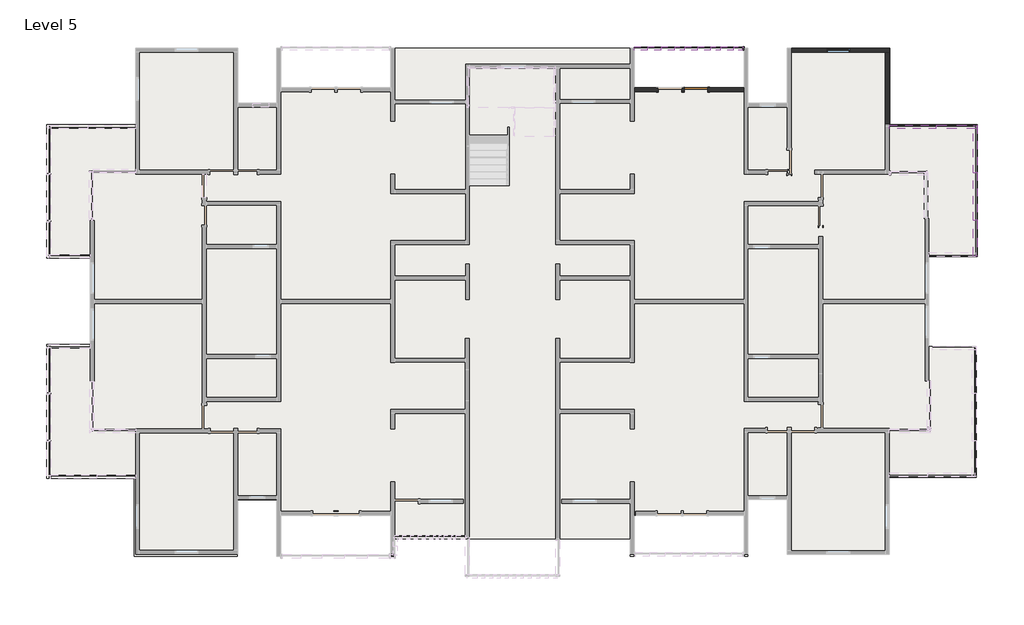
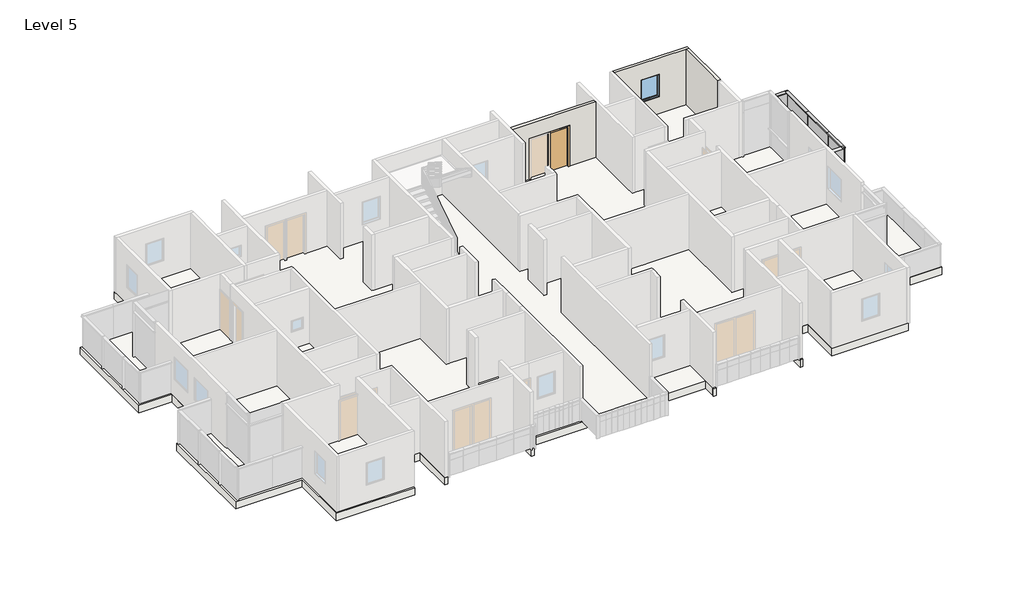
# One storey, part 5 of 7: 15 members, 14 plates, 3 walls, 1 door, 1 slab, 1 window.
"""IFC4 building model written with IfcOpenShell, lengths in millimetres."""

import ifcopenshell
import ifcopenshell.guid

model = None  # the IFC model being written
_history = None  # IfcOwnerHistory: only IFC2X3 demands one
_inside = {}  # id of a spatial element -> (the spatial element, [elements in it])
_under = {}  # id of a project, library or spatial element -> (it, [spatial elements below it])
_declared = {}  # id of a project -> (the project, [libraries it declares])
_typed = {}  # id of a type object -> (the type object, [elements of that type])
_made_of = {}  # id of a material, layer set ... -> (it, [elements and type objects made of it])


def new_model(schema):
    """Start an empty IFC model of exactly this schema.

    Asked for "IFC4X3", IfcOpenShell would pick the latest addendum, in which some entities
    have other attributes; the version numbers below select the first issue.
    IFC2X3 requires an IfcOwnerHistory on every rooted entity: one is made here for all.
    """
    global model, _history
    if schema == "IFC4X3":
        model = ifcopenshell.file(schema_version=(4, 3, 0, 0))
    else:
        model = ifcopenshell.file(schema=schema)
    _inside.clear()
    _under.clear()
    _declared.clear()
    _typed.clear()
    _made_of.clear()
    _history = None
    if model.schema == "IFC2X3":
        org = make("IfcOrganization", Name="unknown")
        user = make(
            "IfcPersonAndOrganization",
            ThePerson=make("IfcPerson", FamilyName="unknown"),
            TheOrganization=org,
        )
        app = make(
            "IfcApplication",
            ApplicationDeveloper=org,
            Version="unknown",
            ApplicationFullName="unknown",
            ApplicationIdentifier="unknown",
        )
        _history = make(
            "IfcOwnerHistory",
            OwningUser=user,
            OwningApplication=app,
            ChangeAction="ADDED",
            CreationDate=0,
        )
    return model


def make(cls, **values):
    """One entity of the class cls with the attributes given. An attribute that is None is left unset."""
    return model.create_entity(
        cls, **{name: value for name, value in values.items() if value is not None}
    )


def rooted(cls, **values):
    """An entity with a GlobalId (a new one), such as an element, a storey or a relation."""
    return make(cls, GlobalId=ifcopenshell.guid.new(), OwnerHistory=_history, **values)


def si_unit(unit_type, name, prefix=None):
    """IfcSIUnit, for example si_unit("LENGTHUNIT", "METRE", prefix="MILLI")."""
    return make("IfcSIUnit", UnitType=unit_type, Prefix=prefix, Name=name)


def assignment(units):
    """IfcUnitAssignment: the units of a project."""
    return None if units is None else make("IfcUnitAssignment", Units=units)


def point(xyz):
    """IfcCartesianPoint."""
    return None if xyz is None else make("IfcCartesianPoint", Coordinates=xyz)


def direction(xyz):
    """IfcDirection."""
    return None if xyz is None else make("IfcDirection", DirectionRatios=xyz)


def frame(location, z_axis=None, x_axis=None):
    """IfcAxis2Placement3D, a coordinate frame: its origin and axes. An axis left out is left unset."""
    return make(
        "IfcAxis2Placement3D",
        Location=point(location),
        Axis=direction(z_axis),
        RefDirection=direction(x_axis),
    )


def origin():
    """The frame at (0, 0, 0) with its axes left unset."""
    return frame((0.0, 0.0, 0.0))


def origin_with_axes():
    """The frame at (0, 0, 0) with the z axis (0, 0, 1) and the x axis (1, 0, 0) written out."""
    return frame((0.0, 0.0, 0.0), z_axis=(0.0, 0.0, 1.0), x_axis=(1.0, 0.0, 0.0))


def place(relative_to, where):
    """IfcLocalPlacement: puts the frame where relative to a parent placement (None: the world)."""
    return make(
        "IfcLocalPlacement", PlacementRelTo=relative_to, RelativePlacement=where
    )


def context(
    kind, dimensions, precision=None, world=None, true_north=None, identifier=None
):
    """IfcGeometricRepresentationContext, for example the 3D "Model" context."""
    return make(
        "IfcGeometricRepresentationContext",
        ContextIdentifier=identifier,
        ContextType=kind,
        CoordinateSpaceDimension=dimensions,
        Precision=precision,
        WorldCoordinateSystem=world,
        TrueNorth=true_north,
    )


def project(units=None, contexts=None):
    """IfcProject with its units and contexts."""
    return rooted(
        "IfcProject",
        Name="project",
        RepresentationContexts=contexts,
        UnitsInContext=assignment(units),
    )


def spatial(cls, under=None, at=None, **own):
    """A site, building, storey or space (cls), placed at a placement, below another one or the project."""
    s = rooted(cls, ObjectPlacement=at, **own)
    if under is not None:
        _under.setdefault(under.id(), (under, []))[1].append(s)
    return s


def polyline(points):
    """IfcPolyline through the points."""
    return make("IfcPolyline", Points=[point(p) for p in points])


def outline(outer, holes=None, kind="AREA"):
    """IfcArbitraryClosedProfileDef: a profile drawn as a closed curve; with holes, ...WithVoids."""
    if holes is None:
        return make("IfcArbitraryClosedProfileDef", ProfileType=kind, OuterCurve=outer)
    return make(
        "IfcArbitraryProfileDefWithVoids",
        ProfileType=kind,
        OuterCurve=outer,
        InnerCurves=holes,
    )


def extrude(swept, where, along, depth):
    """IfcExtrudedAreaSolid: the profile swept, set in the frame where, extruded along a direction by depth."""
    return make(
        "IfcExtrudedAreaSolid",
        SweptArea=swept,
        Position=where,
        ExtrudedDirection=direction(along),
        Depth=depth,
    )


def faces_of(points, faces, orient=None, outer=None):
    """IfcFace entities. A face is a list of loops; a loop is a list of indices into points, from 0.

    orient and outer hold one flag for each loop. By default every Orientation is true, the
    first loop of a face is its IfcFaceOuterBound and the others are IfcFaceBound.
    """
    made = []
    for i, loops in enumerate(faces):
        bounds = []
        for j, loop in enumerate(loops):
            is_outer = j == 0 if outer is None else outer[i][j]
            bounds.append(
                make(
                    "IfcFaceOuterBound" if is_outer else "IfcFaceBound",
                    Bound=make("IfcPolyLoop", Polygon=[points[k] for k in loop]),
                    Orientation=True if orient is None else orient[i][j],
                )
            )
        made.append(make("IfcFace", Bounds=bounds))
    return made


def faceted_brep(points, faces, orient=None, outer=None, voids=None):
    """IfcFacetedBrep: a solid bounded by flat faces; with voids (closed shells), ...WithVoids."""
    shared = [point(p) for p in points]
    hull = make("IfcClosedShell", CfsFaces=faces_of(shared, faces, orient, outer))
    if voids is None:
        return make("IfcFacetedBrep", Outer=hull)
    return make(
        "IfcFacetedBrepWithVoids",
        Outer=hull,
        Voids=[
            make(cls, CfsFaces=faces_of(shared, fs, o, b)) for cls, fs, o, b in voids
        ],
    )


def shape(context_of_items, identifier, shape_type, items):
    """IfcShapeRepresentation: the items that make up one representation, for example the "Body"."""
    return make(
        "IfcShapeRepresentation",
        ContextOfItems=context_of_items,
        RepresentationIdentifier=identifier,
        RepresentationType=shape_type,
        Items=items,
    )


def source(mapping_origin, context_of_items, identifier, shape_type, items):
    """IfcRepresentationMap: a shape defined once, which mapped items show again and again."""
    return make(
        "IfcRepresentationMap",
        MappingOrigin=mapping_origin,
        MappedRepresentation=shape(context_of_items, identifier, shape_type, items),
    )


def transform(
    local_origin,
    x_axis=None,
    y_axis=None,
    z_axis=None,
    scale=None,
    scale2=None,
    scale3=None,
    uniform=True,
):
    """IfcCartesianTransformationOperator3D, or its non-uniform kind. x_axis, y_axis, z_axis: its Axis1, 2, 3."""
    if uniform:
        return make(
            "IfcCartesianTransformationOperator3D",
            Axis1=direction(x_axis),
            Axis2=direction(y_axis),
            LocalOrigin=point(local_origin),
            Scale=scale,
            Axis3=direction(z_axis),
        )
    return make(
        "IfcCartesianTransformationOperator3DnonUniform",
        Axis1=direction(x_axis),
        Axis2=direction(y_axis),
        LocalOrigin=point(local_origin),
        Scale=scale,
        Axis3=direction(z_axis),
        Scale2=scale2,
        Scale3=scale3,
    )


def mapped(mapping_source, mapping_target):
    """IfcMappedItem: shows the shape of a source again, moved by a transform."""
    return make(
        "IfcMappedItem", MappingSource=mapping_source, MappingTarget=mapping_target
    )


def made_of(thing, what):
    """Note that an element or type object is made of a material, layer set ...; save() writes the relation."""
    if what is not None:
        _made_of.setdefault(what.id(), (what, []))[1].append(thing)
    return thing


def element(
    cls,
    number,
    at=None,
    inside=None,
    cuts=None,
    type_object=None,
    material=None,
    context=None,
    identifier="Body",
    shape_type=None,
    held_by="IfcProductDefinitionShape",
    body=None,
    shapes=None,
    **own,
):
    """One element of the class cls, such as IfcWall. Its Tag is "e" and its number.

    at: its placement. inside: the storey or other place that contains it. cuts: it is an
    opening in that element (IfcRelVoidsElement). A single representation is given by context,
    identifier, shape_type and body (its items); several are given by shapes. held_by: the class
    of the entity that holds the representations. save() writes the other relations.
    """
    e = rooted(cls, Tag="e%d" % number, ObjectPlacement=at, **own)
    if body is not None:
        shapes = [shape(context, identifier, shape_type, body)]
    if shapes is not None:
        e.Representation = make(held_by, Representations=shapes)
    if inside is not None:
        _inside.setdefault(inside.id(), (inside, []))[1].append(e)
    if cuts is not None:
        rooted(
            "IfcRelVoidsElement", RelatingBuildingElement=cuts, RelatedOpeningElement=e
        )
    if type_object is not None:
        _typed.setdefault(type_object.id(), (type_object, []))[1].append(e)
    return made_of(e, material)


def aggregate(whole, parts):
    """IfcRelAggregates: a whole, such as a stair, and the parts it consists of."""
    return rooted("IfcRelAggregates", RelatingObject=whole, RelatedObjects=parts)


def save(model, path):
    """Write the relations noted so far, then the file.

    IfcRelAggregates (storeys below a building ...), IfcRelContainedInSpatialStructure (elements
    in a storey), IfcRelDefinesByType, IfcRelAssociatesMaterial and IfcRelDeclares: one each for
    every whole, place, type object, material and project.
    """
    for whole, parts in _under.values():
        aggregate(whole, parts)
    for where, things in _inside.values():
        rooted(
            "IfcRelContainedInSpatialStructure",
            RelatedElements=things,
            RelatingStructure=where,
        )
    for kind, things in _typed.values():
        rooted("IfcRelDefinesByType", RelatedObjects=things, RelatingType=kind)
    for what, things in _made_of.values():
        rooted("IfcRelAssociatesMaterial", RelatedObjects=things, RelatingMaterial=what)
    for by, libraries in _declared.values():
        rooted("IfcRelDeclares", RelatingContext=by, RelatedDefinitions=libraries)
    model.write(path)


def m_single_flush_0915_x_2134mm_138fd904(model_context):
    return source(origin(), model_context, "Body", "SweptSolid", [
        extrude(outline(polyline([(2210.0, -533.5), (0.0, -533.5), (0.0, -457.5), (2134.0, -457.5), (2134.0, 457.5), (0.0, 457.5), (0.0, 533.5), (2210.0, 533.5), (2210.0, -533.5)])), frame((0.0, 75.0, 0.0), z_axis=(0.0, 1.0, 0.0), x_axis=(0.0, 0.0, 1.0)), (0.0, 0.0, 1.0), 25.0),
        extrude(outline(polyline([(2210.0, 533.5), (2210.0, -533.5), (0.0, -533.5), (0.0, -457.5), (2134.0, -457.5), (2134.0, 457.5), (0.0, 457.5), (0.0, 533.5), (2210.0, 533.5)])), frame((0.0, -100.0, 0.0), z_axis=(0.0, 1.0, 0.0), x_axis=(0.0, 0.0, 1.0)), (0.0, 0.0, 1.0), 25.0),
        extrude(outline(polyline([(457.5, 24.0), (-457.5, 24.0), (-457.5, 75.0), (457.5, 75.0), (457.5, 24.0)])), origin_with_axes(), (0.0, 0.0, 1.0), 2134.0),
    ])


def rectangular_mullion_50mm_x_150mm_42770ee2(model_context):
    return source(origin(), model_context, "Body", "SweptSolid", [
        extrude(outline(polyline([(0.0, 75.0), (0.0, -75.0), (-50.0, -75.0), (-50.0, 75.0), (0.0, 75.0)])), frame((0.0, 0.0, -1830.0000003), z_axis=(0.0, 0.0, 1.0), x_axis=(1.0, 0.0, 0.0)), (0.0, 0.0, 1.0), 1830.0000003),
    ])


def rectangular_mullion_50mm_x_150mm_aaee7d48(model_context):
    return source(origin(), model_context, "Body", "SweptSolid", [
        extrude(outline(polyline([(0.0, 75.0), (0.0, -75.0), (-50.0, -75.0), (-50.0, 75.0), (0.0, 75.0)])), frame((0.0, 0.0, -1830.0), z_axis=(0.0, 0.0, 1.0), x_axis=(1.0, 0.0, 0.0)), (0.0, 0.0, 1.0), 1830.0),
    ])


def rectangular_mullion_50mm_x_150mm_efa02866(model_context):
    return source(origin(), model_context, "Body", "SweptSolid", [
        extrude(outline(polyline([(0.0, 75.0), (0.0, -75.0), (-50.0, -75.0), (-50.0, 75.0), (0.0, 75.0)])), frame((0.0, 0.0, -1399.9999997), z_axis=(0.0, 0.0, 1.0), x_axis=(1.0, 0.0, 0.0)), (0.0, 0.0, 1.0), 1399.9999997),
    ])


def rectangular_mullion_50mm_x_150mm_d9f1e9e9(model_context):
    return source(origin(), model_context, "Body", "SweptSolid", [
        extrude(outline(polyline([(0.0, 75.0), (0.0, -75.0), (-50.0, -75.0), (-50.0, 75.0), (0.0, 75.0)])), frame((0.0, 0.0, -1565.8160321), z_axis=(0.0, 0.0, 1.0), x_axis=(1.0, 0.0, 0.0)), (0.0, 0.0, 1.0), 1565.8160321),
    ])


def rectangular_mullion_50mm_x_150mm_729c0cfc(model_context):
    return source(origin(), model_context, "Body", "SweptSolid", [
        extrude(outline(polyline([(0.0, 75.0), (0.0, -75.0), (-50.0, -75.0), (-50.0, 75.0), (0.0, 75.0)])), frame((0.0, 0.0, -1250.0), z_axis=(0.0, 0.0, 1.0), x_axis=(1.0, 0.0, 0.0)), (0.0, 0.0, 1.0), 1250.0),
    ])


def rectangular_mullion_50mm_x_150mm_b3666dbd(model_context):
    return source(origin(), model_context, "Body", "SweptSolid", [
        extrude(outline(polyline([(0.0, 75.0), (0.0, -75.0), (-50.0, -75.0), (-50.0, 75.0), (0.0, 75.0)])), frame((0.0, 0.0, -500.0), z_axis=(0.0, 0.0, 1.0), x_axis=(1.0, 0.0, 0.0)), (0.0, 0.0, 1.0), 500.0),
    ])


def rectangular_mullion_50mm_x_150mm_e851a0b8(model_context):
    return source(origin(), model_context, "Body", "SweptSolid", [
        extrude(outline(polyline([(0.0, 75.0), (0.0, -75.0), (-50.0, -75.0), (-50.0, 75.0), (0.0, 75.0)])), frame((0.0, 0.0, -522.7272727), z_axis=(0.0, 0.0, 1.0), x_axis=(1.0, 0.0, 0.0)), (0.0, 0.0, 1.0), 522.7272727),
    ])


def rectangular_mullion_50mm_x_150mm_e11a3e7b(model_context):
    return source(origin(), model_context, "Body", "SweptSolid", [
        extrude(outline(polyline([(0.0, 75.0), (0.0, -75.0), (-50.0, -75.0), (-50.0, 75.0), (0.0, 75.0)])), frame((0.0, 0.0, -400.0), z_axis=(0.0, 0.0, 1.0), x_axis=(1.0, 0.0, 0.0)), (0.0, 0.0, 1.0), 400.0),
    ])


def rectangular_mullion_50mm_x_150mm_23485ade(model_context):
    return source(origin(), model_context, "Body", "SweptSolid", [
        extrude(outline(polyline([(0.0, 75.0), (0.0, -75.0), (-50.0, -75.0), (-50.0, 75.0), (0.0, 75.0)])), frame((0.0, 0.0, -350.0), z_axis=(0.0, 0.0, 1.0), x_axis=(1.0, 0.0, 0.0)), (0.0, 0.0, 1.0), 350.0),
    ])


def system_panel_glazed_09fbcc53(model_context):
    return source(origin(), model_context, "Body", "SweptSolid", [
        extrude(outline(polyline([(915.0000002, 24.5), (-915.0000002, 24.5), (-915.0000002, 49.5), (915.0000002, 49.5), (915.0000002, 24.5)])), origin_with_axes(), (0.0, 0.0, 1.0), 1200.0),
    ])


def system_panel_glazed_f4bbd109(model_context):
    return source(origin(), model_context, "Body", "SweptSolid", [
        extrude(outline(polyline([(910.8343113, 24.5), (-910.8343113, 24.5), (-910.8343113, 49.5), (910.8343113, 49.5), (910.8343113, 24.5)])), origin_with_axes(), (0.0, 0.0, 1.0), 1200.0),
    ])


def system_panel_glazed_42eec186(model_context):
    return source(origin(), model_context, "Body", "SweptSolid", [
        extrude(outline(polyline([(699.9999998, 24.5), (-699.9999998, 24.5), (-699.9999998, 49.5), (699.9999998, 49.5), (699.9999998, 24.5)])), origin_with_axes(), (0.0, 0.0, 1.0), 1200.0),
    ])


def system_panel_glazed_f2fc581d(model_context):
    return source(origin(), model_context, "Body", "SweptSolid", [
        extrude(outline(polyline([(782.9080161, 24.5), (-782.9080161, 24.5), (-782.9080161, 49.5), (782.9080161, 49.5), (782.9080161, 24.5)])), origin_with_axes(), (0.0, 0.0, 1.0), 1200.0),
    ])


def system_panel_glazed_346501af(model_context):
    return source(origin(), model_context, "Body", "SweptSolid", [
        extrude(outline(polyline([(250.0, 24.5), (-250.0, 24.5), (-250.0, 49.5), (250.0, 49.5), (250.0, 24.5)])), origin_with_axes(), (0.0, 0.0, 1.0), 1200.0),
    ])


def system_panel_glazed_5241e6d5(model_context):
    return source(origin(), model_context, "Body", "SweptSolid", [
        extrude(outline(polyline([(261.3636364, 24.5), (-261.3636364, 24.5), (-261.3636364, 49.5), (261.3636364, 49.5), (261.3636364, 24.5)])), origin_with_axes(), (0.0, 0.0, 1.0), 1200.0),
    ])


def system_panel_glazed_3e660766(model_context):
    return source(origin(), model_context, "Body", "SweptSolid", [
        extrude(outline(polyline([(200.0, 24.5), (-200.0, 24.5), (-200.0, 49.5), (200.0, 49.5), (200.0, 24.5)])), origin_with_axes(), (0.0, 0.0, 1.0), 1200.0),
    ])


def system_panel_glazed_b0a6d7cd(model_context):
    return source(origin(), model_context, "Body", "SweptSolid", [
        extrude(outline(polyline([(175.0, 24.5), (-175.0, 24.5), (-175.0, 49.5), (175.0, 49.5), (175.0, 24.5)])), origin_with_axes(), (0.0, 0.0, 1.0), 1200.0),
    ])


def m_fixed_0915_x_1220mm_873aa0e2(model_context):
    return source(origin(), model_context, "Body", "SweptSolid", [
        extrude(outline(polyline([(-394.5, 53.0), (394.5, 53.0), (394.5, 41.0), (-394.5, 41.0), (-394.5, 53.0)])), frame((0.0, 0.0, 978.0), z_axis=(0.0, 0.0, 1.0), x_axis=(1.0, 0.0, 0.0)), (0.0, 0.0, 1.0), 1094.0),
        extrude(outline(polyline([(2116.0, -438.5), (934.0, -438.5), (934.0, 438.5), (2116.0, 438.5), (2116.0, -438.5)]), holes=[polyline([(2072.0, -394.5), (2072.0, 394.5), (978.0, 394.5), (978.0, -394.5), (2072.0, -394.5)])]), frame((0.0, 25.0, 0.0), z_axis=(0.0, 1.0, 0.0), x_axis=(0.0, 0.0, 1.0)), (0.0, 0.0, 1.0), 44.0),
        extrude(outline(polyline([(2135.0, -457.5), (915.0, -457.5), (915.0, 457.5), (2135.0, 457.5), (2135.0, -457.5)]), holes=[polyline([(2116.0, -438.5), (2116.0, 438.5), (934.0, 438.5), (934.0, -438.5), (2116.0, -438.5)])]), frame((0.0, 25.0, 0.0), z_axis=(0.0, 1.0, 0.0), x_axis=(0.0, 0.0, 1.0)), (0.0, 0.0, 1.0), 63.0),
        extrude(outline(polyline([(2135.0, -457.5), (915.0, -457.5), (915.0, 457.5), (2135.0, 457.5), (2135.0, -457.5)]), holes=[polyline([(2103.0, -425.5), (2103.0, 425.5), (947.0, 425.5), (947.0, -425.5), (2103.0, -425.5)])]), frame((0.0, -62.0, 0.0), z_axis=(0.0, 1.0, 0.0), x_axis=(0.0, 0.0, 1.0)), (0.0, 0.0, 1.0), 87.0),
    ])


model = new_model("IFC4")

# Units and contexts
model_context = context("Model", 3, world=origin())
ifc_project = project(units=[si_unit("LENGTHUNIT", "METRE", prefix="MILLI")], contexts=[model_context])

# Site, building, storey
site = spatial("IfcSite", under=ifc_project)
building = spatial("IfcBuilding", under=site)
storey = spatial("IfcBuildingStorey", under=building, Name="Level 5", Elevation=12500.0)

# Door
placement = place(None, origin())
m_single_flush_0915_x_2134mm_shape = m_single_flush_0915_x_2134mm_138fd904(model_context)
element("IfcDoor", 1, ObjectType="M_Single-Flush : 0915 x 2134mm", at=placement, inside=storey, context=model_context, shape_type="MappedRepresentation", body=[
    mapped(m_single_flush_0915_x_2134mm_shape, transform((6794.6515415, 8016.5690894, 12500.0), x_axis=(1.0, 0.0, 0.0), y_axis=(0.0, 1.0, 0.0), z_axis=(0.0, 0.0, 1.0))),
])

# Members
rectangular_mullion_50mm_x_150mm_shape = rectangular_mullion_50mm_x_150mm_42770ee2(model_context)
element("IfcMember", 2, ObjectType="Rectangular Mullion : 50mm x 150mm", at=placement, inside=storey, context=model_context, shape_type="MappedRepresentation", body=[
    mapped(rectangular_mullion_50mm_x_150mm_shape, transform((17635.0130284, 4788.3418163, 13750.0), x_axis=(0.0, 0.0, 1.0), y_axis=(-1.0, 0.0, 0.0), z_axis=(0.0, -1.0, 0.0))),
])
element("IfcMember", 3, ObjectType="Rectangular Mullion : 50mm x 150mm", at=placement, inside=storey, context=model_context, shape_type="MappedRepresentation", body=[
    mapped(rectangular_mullion_50mm_x_150mm_shape, transform((16129.1969963, 6568.8418166, 13750.0), x_axis=(0.0, 0.0, 1.0), y_axis=(0.0, -1.0, 0.0), z_axis=(1.0, 0.0, 0.0))),
])
rectangular_mullion_50mm_x_150mm_2_shape = rectangular_mullion_50mm_x_150mm_aaee7d48(model_context)
element("IfcMember", 4, ObjectType="Rectangular Mullion : 50mm x 150mm", at=placement, inside=storey, context=model_context, shape_type="MappedRepresentation", body=[
    mapped(rectangular_mullion_50mm_x_150mm_2_shape, transform((17635.0130284, 2958.3418163, 13750.0), x_axis=(0.0, 0.0, 1.0), y_axis=(-1.0, 0.0, 0.0), z_axis=(0.0, -1.0, 0.0))),
])
rectangular_mullion_50mm_x_150mm_3_shape = rectangular_mullion_50mm_x_150mm_efa02866(model_context)
element("IfcMember", 5, ObjectType="Rectangular Mullion : 50mm x 150mm", at=placement, inside=storey, context=model_context, shape_type="MappedRepresentation", body=[
    mapped(rectangular_mullion_50mm_x_150mm_3_shape, transform((17635.0130284, 1558.3418166, 13750.0), x_axis=(0.0, 0.0, 1.0), y_axis=(-1.0, 0.0, 0.0), z_axis=(0.0, -1.0, 0.0))),
])
rectangular_mullion_50mm_x_150mm_4_shape = rectangular_mullion_50mm_x_150mm_d9f1e9e9(model_context)
element("IfcMember", 6, ObjectType="Rectangular Mullion : 50mm x 150mm", at=placement, inside=storey, context=model_context, shape_type="MappedRepresentation", body=[
    mapped(rectangular_mullion_50mm_x_150mm_4_shape, transform((17695.0130284, 6568.8418166, 13750.0), x_axis=(0.0, 0.0, 1.0), y_axis=(0.0, -1.0, 0.0), z_axis=(1.0, 0.0, 0.0))),
])
rectangular_mullion_50mm_x_150mm_5_shape = rectangular_mullion_50mm_x_150mm_729c0cfc(model_context)
element("IfcMember", 7, ObjectType="Rectangular Mullion : 50mm x 150mm", at=placement, inside=storey, context=model_context, shape_type="MappedRepresentation", body=[
    mapped(rectangular_mullion_50mm_x_150mm_5_shape, transform((8667.3788142, 9614.2963621, 12500.0), x_axis=(1.0, 0.0, 0.0), y_axis=(0.0, -1.0, 0.0), z_axis=(0.0, 0.0, -1.0))),
])
rectangular_mullion_50mm_x_150mm_6_shape = rectangular_mullion_50mm_x_150mm_b3666dbd(model_context)
element("IfcMember", 8, ObjectType="Rectangular Mullion : 50mm x 150mm", at=placement, inside=storey, context=model_context, shape_type="MappedRepresentation", body=[
    mapped(rectangular_mullion_50mm_x_150mm_6_shape, transform((6867.3788142, 9614.2963621, 13750.0), x_axis=(0.0, 0.0, 1.0), y_axis=(0.0, -1.0, 0.0), z_axis=(1.0, 0.0, 0.0))),
])
element("IfcMember", 9, ObjectType="Rectangular Mullion : 50mm x 150mm", at=placement, inside=storey, context=model_context, shape_type="MappedRepresentation", body=[
    mapped(rectangular_mullion_50mm_x_150mm_6_shape, transform((7367.3788142, 9614.2963621, 13750.0), x_axis=(0.0, 0.0, 1.0), y_axis=(0.0, -1.0, 0.0), z_axis=(1.0, 0.0, 0.0))),
])
element("IfcMember", 10, ObjectType="Rectangular Mullion : 50mm x 150mm", at=placement, inside=storey, context=model_context, shape_type="MappedRepresentation", body=[
    mapped(rectangular_mullion_50mm_x_150mm_6_shape, transform((8267.3788142, 9614.2963621, 13750.0), x_axis=(0.0, 0.0, 1.0), y_axis=(0.0, -1.0, 0.0), z_axis=(1.0, 0.0, 0.0))),
])
rectangular_mullion_50mm_x_150mm_7_shape = rectangular_mullion_50mm_x_150mm_e851a0b8(model_context)
element("IfcMember", 11, ObjectType="Rectangular Mullion : 50mm x 150mm", at=placement, inside=storey, context=model_context, shape_type="MappedRepresentation", body=[
    mapped(rectangular_mullion_50mm_x_150mm_7_shape, transform((4921.9242687, 9614.2963621, 13750.0), x_axis=(0.0, 0.0, 1.0), y_axis=(0.0, -1.0, 0.0), z_axis=(1.0, 0.0, 0.0))),
])
element("IfcMember", 12, ObjectType="Rectangular Mullion : 50mm x 150mm", at=placement, inside=storey, context=model_context, shape_type="MappedRepresentation", body=[
    mapped(rectangular_mullion_50mm_x_150mm_7_shape, transform((5444.6515415, 9614.2963621, 13750.0), x_axis=(0.0, 0.0, 1.0), y_axis=(0.0, -1.0, 0.0), z_axis=(1.0, 0.0, 0.0))),
])
element("IfcMember", 13, ObjectType="Rectangular Mullion : 50mm x 150mm", at=placement, inside=storey, context=model_context, shape_type="MappedRepresentation", body=[
    mapped(rectangular_mullion_50mm_x_150mm_7_shape, transform((5967.3788142, 9614.2963621, 13750.0), x_axis=(0.0, 0.0, 1.0), y_axis=(0.0, -1.0, 0.0), z_axis=(1.0, 0.0, 0.0))),
])
rectangular_mullion_50mm_x_150mm_8_shape = rectangular_mullion_50mm_x_150mm_e11a3e7b(model_context)
element("IfcMember", 14, ObjectType="Rectangular Mullion : 50mm x 150mm", at=placement, inside=storey, context=model_context, shape_type="MappedRepresentation", body=[
    mapped(rectangular_mullion_50mm_x_150mm_8_shape, transform((6367.3788142, 9614.2963621, 13750.0), x_axis=(0.0, 0.0, 1.0), y_axis=(0.0, -1.0, 0.0), z_axis=(1.0, 0.0, 0.0))),
])
element("IfcMember", 15, ObjectType="Rectangular Mullion : 50mm x 150mm", at=placement, inside=storey, context=model_context, shape_type="MappedRepresentation", body=[
    mapped(rectangular_mullion_50mm_x_150mm_8_shape, transform((7767.3788142, 9614.2963621, 13750.0), x_axis=(0.0, 0.0, 1.0), y_axis=(0.0, -1.0, 0.0), z_axis=(1.0, 0.0, 0.0))),
])
rectangular_mullion_50mm_x_150mm_9_shape = rectangular_mullion_50mm_x_150mm_23485ade(model_context)
element("IfcMember", 16, ObjectType="Rectangular Mullion : 50mm x 150mm", at=placement, inside=storey, context=model_context, shape_type="MappedRepresentation", body=[
    mapped(rectangular_mullion_50mm_x_150mm_9_shape, transform((8617.3788142, 9614.2963621, 13750.0), x_axis=(0.0, 0.0, 1.0), y_axis=(0.0, -1.0, 0.0), z_axis=(1.0, 0.0, 0.0))),
])

# Plates
system_panel_glazed_shape = system_panel_glazed_09fbcc53(model_context)
element("IfcPlate", 17, ObjectType="System Panel : Glazed", at=placement, inside=storey, context=model_context, shape_type="MappedRepresentation", body=[
    mapped(system_panel_glazed_shape, transform((17635.0130284, 5703.3418165, 12500.0), x_axis=(0.0, -1.0, 0.0), y_axis=(1.0, 0.0, 0.0), z_axis=(0.0, 0.0, 1.0))),
])
element("IfcPlate", 18, ObjectType="System Panel : Glazed", at=placement, inside=storey, context=model_context, shape_type="MappedRepresentation", body=[
    mapped(system_panel_glazed_shape, transform((17635.0130284, 3873.3418163, 12500.0), x_axis=(0.0, -1.0, 0.0), y_axis=(1.0, 0.0, 0.0), z_axis=(0.0, 0.0, 1.0))),
])
system_panel_glazed_2_shape = system_panel_glazed_f4bbd109(model_context)
element("IfcPlate", 19, ObjectType="System Panel : Glazed", at=placement, inside=storey, context=model_context, shape_type="MappedRepresentation", body=[
    mapped(system_panel_glazed_2_shape, transform((16748.6787171, 1608.3418166, 12500.0), x_axis=(-1.0, 0.0, 0.0), y_axis=(0.0, -1.0, 0.0), z_axis=(0.0, 0.0, 1.0))),
])
system_panel_glazed_3_shape = system_panel_glazed_42eec186(model_context)
element("IfcPlate", 20, ObjectType="System Panel : Glazed", at=placement, inside=storey, context=model_context, shape_type="MappedRepresentation", body=[
    mapped(system_panel_glazed_3_shape, transform((17635.0130284, 2258.3418165, 12500.0), x_axis=(0.0, -1.0, 0.0), y_axis=(1.0, 0.0, 0.0), z_axis=(0.0, 0.0, 1.0))),
])
system_panel_glazed_4_shape = system_panel_glazed_f2fc581d(model_context)
element("IfcPlate", 21, ObjectType="System Panel : Glazed", at=placement, inside=storey, context=model_context, shape_type="MappedRepresentation", body=[
    mapped(system_panel_glazed_4_shape, transform((16912.1050124, 6568.8418166, 12500.0), x_axis=(1.0, 0.0, 0.0), y_axis=(0.0, 1.0, 0.0), z_axis=(0.0, 0.0, 1.0))),
])
system_panel_glazed_5_shape = system_panel_glazed_346501af(model_context)
element("IfcPlate", 22, ObjectType="System Panel : Glazed", at=placement, inside=storey, context=model_context, shape_type="MappedRepresentation", body=[
    mapped(system_panel_glazed_5_shape, transform((8017.3788142, 9614.2963621, 12500.0), x_axis=(1.0, 0.0, 0.0), y_axis=(0.0, 1.0, 0.0), z_axis=(0.0, 0.0, 1.0))),
])
element("IfcPlate", 23, ObjectType="System Panel : Glazed", at=placement, inside=storey, context=model_context, shape_type="MappedRepresentation", body=[
    mapped(system_panel_glazed_5_shape, transform((7117.3788142, 9614.2963621, 12500.0), x_axis=(1.0, 0.0, 0.0), y_axis=(0.0, 1.0, 0.0), z_axis=(0.0, 0.0, 1.0))),
])
element("IfcPlate", 24, ObjectType="System Panel : Glazed", at=placement, inside=storey, context=model_context, shape_type="MappedRepresentation", body=[
    mapped(system_panel_glazed_5_shape, transform((6617.3788142, 9614.2963621, 12500.0), x_axis=(1.0, 0.0, 0.0), y_axis=(0.0, 1.0, 0.0), z_axis=(0.0, 0.0, 1.0))),
])
system_panel_glazed_6_shape = system_panel_glazed_5241e6d5(model_context)
element("IfcPlate", 25, ObjectType="System Panel : Glazed", at=placement, inside=storey, context=model_context, shape_type="MappedRepresentation", body=[
    mapped(system_panel_glazed_6_shape, transform((4660.5606324, 9614.2963621, 12500.0), x_axis=(1.0, 0.0, 0.0), y_axis=(0.0, 1.0, 0.0), z_axis=(0.0, 0.0, 1.0))),
])
element("IfcPlate", 26, ObjectType="System Panel : Glazed", at=placement, inside=storey, context=model_context, shape_type="MappedRepresentation", body=[
    mapped(system_panel_glazed_6_shape, transform((5706.0151778, 9614.2963621, 12500.0), x_axis=(1.0, 0.0, 0.0), y_axis=(0.0, 1.0, 0.0), z_axis=(0.0, 0.0, 1.0))),
])
element("IfcPlate", 27, ObjectType="System Panel : Glazed", at=placement, inside=storey, context=model_context, shape_type="MappedRepresentation", body=[
    mapped(system_panel_glazed_6_shape, transform((5183.2879051, 9614.2963621, 12500.0), x_axis=(1.0, 0.0, 0.0), y_axis=(0.0, 1.0, 0.0), z_axis=(0.0, 0.0, 1.0))),
])
system_panel_glazed_7_shape = system_panel_glazed_3e660766(model_context)
element("IfcPlate", 28, ObjectType="System Panel : Glazed", at=placement, inside=storey, context=model_context, shape_type="MappedRepresentation", body=[
    mapped(system_panel_glazed_7_shape, transform((7567.3788142, 9614.2963621, 12500.0), x_axis=(1.0, 0.0, 0.0), y_axis=(0.0, 1.0, 0.0), z_axis=(0.0, 0.0, 1.0))),
])
element("IfcPlate", 29, ObjectType="System Panel : Glazed", at=placement, inside=storey, context=model_context, shape_type="MappedRepresentation", body=[
    mapped(system_panel_glazed_7_shape, transform((6167.3788142, 9614.2963621, 12500.0), x_axis=(1.0, 0.0, 0.0), y_axis=(0.0, 1.0, 0.0), z_axis=(0.0, 0.0, 1.0))),
])
system_panel_glazed_8_shape = system_panel_glazed_b0a6d7cd(model_context)
element("IfcPlate", 30, ObjectType="System Panel : Glazed", at=placement, inside=storey, context=model_context, shape_type="MappedRepresentation", body=[
    mapped(system_panel_glazed_8_shape, transform((8442.3788142, 9614.2963621, 12500.0), x_axis=(1.0, 0.0, 0.0), y_axis=(0.0, 1.0, 0.0), z_axis=(0.0, 0.0, 1.0))),
])

# Slab
element("IfcSlab", 31, ObjectType="Generic Floor - 400mm", at=placement, inside=storey, context=model_context, shape_type="SweptSolid", body=[
    extrude(outline(polyline([(-10978.0757313, 7482.4781803), (-9455.3484585, 7482.4781803), (-9455.3484585, 9614.2963621), (-9305.3484585, 9614.2963621), (-9305.3484585, 8091.5690894), (-5039.4393676, 8091.5690894), (-5039.4393676, 9614.2963621), (4399.196996, 9614.2963621), (4399.196996, 8091.5690894), (8665.1060869, 8091.5690894), (8665.1060869, 9614.2963621), (8817.3788142, 9614.2963621), (8817.3788142, 7482.4781803), (10342.3783683, 7482.4781803), (10342.3783683, 9614.2963621), (14312.8444058, 9614.2963621), (14312.8444058, 6653.3418166), (17717.8444058, 6653.3418166), (17717.8444058, 1533.3418166), (15837.8444058, 1533.3418166), (15837.8444058, -1946.1581834), (17677.8444058, -1946.1581834), (17677.8444058, -7028.8854561), (14240.1060869, -7028.8854561), (14240.1060869, -10028.8854561), (10340.1060869, -10028.8854561), (10340.1060869, -7894.794547), (8815.1060869, -7894.794547), (8815.1060869, -10106.1581834), (8665.1060869, -10106.1581834), (8665.1060869, -8506.1581834), (4401.4697233, -8506.1581834), (4401.4697233, -10106.1581834), (4251.4697233, -10106.1581834), (4251.4697233, -10028.8854561), (4251.4697233, -9417.5218198), (-4887.1666404, -9417.5218198), (-4887.1666404, -10006.7413208), (-4887.1666404, -10106.1581834), (-5039.4393676, -10106.1581834), (-5039.4393676, -8503.8854561), (-9303.0757313, -8503.8854561), (-9303.0757313, -10106.1581834), (-9453.0757313, -10106.1581834), (-9453.0757313, -7906.1581834), (-10989.3512663, -7906.1581834), (-10989.3512663, -10106.1581834), (-14989.3512663, -10106.1581834), (-14989.3512663, -7083.4309107), (-18389.3512663, -7083.4309107), (-18389.3512663, -1883.4309107), (-16697.1666404, -1883.4309107), (-16697.1666404, 1474.2963621), (-18377.1666404, 1474.2963621), (-18377.1666404, 6654.2963621), (-14937.1666404, 6654.2963621), (-14937.1666404, 9614.2963621), (-10978.0757313, 9614.2963621), (-10978.0757313, 7482.4781803)])), frame((0.0, 0.0, 12100.0), z_axis=(0.0, 0.0, 1.0), x_axis=(1.0, 0.0, 0.0)), (0.0, 0.0, 1.0), 400.0),
])

# Walls
element("IfcWall", 32, ObjectType="wal 150", at=placement, inside=storey, context=model_context, shape_type="SweptSolid", body=[
    extrude(outline(polyline([(12500.0, 8665.1060869), (15500.0, 8665.1060869), (15500.0, 4399.196996), (12500.0, 4399.196996), (12500.0, 5337.1515415), (14634.0, 5337.1515415), (14634.0, 6252.1515415), (12500.0, 6252.1515415), (12500.0, 6337.1515415), (14634.0, 6337.1515415), (14634.0, 7252.1515415), (12500.0, 7252.1515415), (12500.0, 8665.1060869)])), frame((0.0, 7941.5690894, 0.0), z_axis=(0.0, 1.0, 0.0), x_axis=(0.0, 0.0, 1.0)), (0.0, 0.0, 1.0), 150.0),
])
element("IfcWall", 33, ObjectType="wal 150", at=placement, inside=storey, context=model_context, shape_type="Brep", body=[
    faceted_brep([(10492.3783683, 9464.2963621, 12500.0), (14149.196996, 9464.2963621, 12500.0), (14299.196996, 9464.2963621, 12500.0), (14299.196996, 9464.2963621, 15500.0), (14149.196996, 9464.2963621, 15500.0), (10492.3783683, 9464.2963621, 15500.0), (11863.2876822, 9464.2963621, 13415.0), (11863.2876822, 9464.2963621, 14635.0), (12778.2876822, 9464.2963621, 14635.0), (12778.2876822, 9464.2963621, 13415.0), (10492.3783683, 9614.2963621, 12500.0), (10492.3783683, 9614.2963621, 15500.0), (14299.196996, 9614.2963621, 15500.0), (14299.196996, 9614.2963621, 12500.0), (11863.2876822, 9614.2963621, 13415.0), (12778.2876822, 9614.2963621, 13415.0), (12778.2876822, 9614.2963621, 14635.0), (11863.2876822, 9614.2963621, 14635.0)], [[[0, 1, 2, 3, 4, 5], [6, 7, 8, 9]], [[10, 11, 12, 13], [14, 15, 16, 17]], [[2, 1, 0, 10, 13]], [[5, 4, 3, 12, 11]], [[7, 6, 14, 17]], [[8, 7, 17, 16]], [[9, 8, 16, 15]], [[6, 9, 15, 14]], [[0, 5, 11, 10]], [[3, 2, 13, 12]]]),
])
element("IfcWall", 34, ObjectType="wal 150", at=placement, inside=storey, context=model_context, shape_type="SweptSolid", body=[
    extrude(outline(polyline([(14149.196996, 6668.8418166), (14149.196996, 9464.2963621), (14299.196996, 9464.2963621), (14299.196996, 6668.8418166), (14149.196996, 6668.8418166)])), frame((0.0, 0.0, 12500.0), z_axis=(0.0, 0.0, 1.0), x_axis=(1.0, 0.0, 0.0)), (0.0, 0.0, 1.0), 3000.0),
])

# Window
m_fixed_0915_x_1220mm_shape = m_fixed_0915_x_1220mm_873aa0e2(model_context)
element("IfcWindow", 35, ObjectType="M_Fixed : 1.80 to 1.20 w2", at=placement, inside=storey, context=model_context, shape_type="MappedRepresentation", body=[
    mapped(m_fixed_0915_x_1220mm_shape, transform((12320.7876822, 9526.2963621, 12500.0), x_axis=(1.0, 0.0, 0.0), y_axis=(0.0, 1.0, 0.0), z_axis=(0.0, 0.0, 1.0))),
])

save(model, "model.ifc")

# Revit data of these elements
# Type "M_Single-Flush : 0915 x 2134mm"
#   Type Mark = "15"
#   Thickness = 0.051 m
#   Height = 2.134 m
#   Trim Projection Ext = 0.025 m
#   Trim Projection Int = 0.025 m
#   Trim Width = 0.076 m
#   Width = 0.915 m
#   Door Material = Door - Panel
#   Frame Material = Door - Frame
#   Function = (empty or 0)
#   Wall Closure = (empty or 0)
# Type "Rectangular Mullion : 50mm x 150mm"
#   built-in parameter 1007304 = 0.492126 (stored number, unit not read)
#   built-in parameter 1007301 = 0.082021 (stored number, unit not read)
#   built-in parameter 1007300 = 0.082021 (stored number, unit not read)
# Type "Generic Floor - 400mm"
#   Function = 0
#   Layers, outside or top first: 0.4 m no material (function 1)
# Type "wal 150"
#   Layers, outside or top first: 0.15 m no material (function 1)
# Type "M_Fixed : 1.80 to 1.20 w2"
#   Type Mark = "19"
#   Height = 1.22 m
#   Default Sill Height = 0.915 m
#   Width = 0.915 m
#   Window Inset = 0.019 m
#   Frame Exterior Material = Sash
#   Frame Interior Material = Sash
#   Glass Pane Material = Glass
#   Sash = Sash
#   Wall Closure = (empty or 0)
# Element 1 (IfcDoor, "M_Single-Flush : 0915 x 2134mm")
#   Phase Created = New Construction
#   Materials on its faces: "Door - Frame", "Door - Panel"
# Elements 2, 3, 4, 5, 6, 7, 8, 9, 10, 11, 12, 13, 14, 15, 16 (IfcMember, "Rectangular Mullion : 50mm x 150mm")
#   Phase Created = New Construction
#   Materials on its faces: "Aluminum"
# Elements 17, 18, 19, 20, 21, 22, 23, 24, 25, 26, 27, 28, 29, 30 (IfcPlate, "System Panel : Glazed")
#   Phase Created = New Construction
#   Materials on its faces: "Glass"
# Element 31 (IfcSlab, "Generic Floor - 400mm")
#   built-in parameter 1001955 = 3.14159 (stored number, unit not read)
#   Height Offset From Level = 0 m
#   Phase Created = New Construction
#   Materials on its faces: "Default Roof", "Door - Frame", "Ceiling Tile 600 x 1200", "Oak Flooring"
# Element 32 (IfcWall, "wal 150")
#   Top Offset = 0 m
#   Base Offset = 0 m
#   Unconnected Height = 3 m
#   wall height = 3 m
#   Phase Created = New Construction
#   Base Constraint = Level 5
#   Materials on its faces: "Default Wall", "Door - Frame"
# Element 33 (IfcWall, "wal 150")
#   Top Offset = 0 m
#   Base Offset = 0 m
#   Unconnected Height = 3 m
#   wall height = 3 m
#   Phase Created = New Construction
#   Base Constraint = Level 5
#   Materials on its faces: "Default Wall", "Ceiling Tile 600 x 600", "Ceiling Tile 600 x 1200"
# Element 34 (IfcWall, "wal 150")
#   Top Offset = 0 m
#   Base Offset = 0 m
#   Unconnected Height = 3 m
#   wall height = 3 m
#   Phase Created = New Construction
#   Base Constraint = Level 5
#   Materials on its faces: "Default Wall", "Ceiling Tile 600 x 1200"
# Element 35 (IfcWindow, "M_Fixed : 1.80 to 1.20 w2")
#   Mark = "351"
#   Phase Created = New Construction
#   Materials on its faces: "Sash", "Glass"
# Materials
#   "Door - Panel": class "Wood", colour RGB 114 82 51, transparency 0
#   "Door - Frame": class "Miscellaneous", colour RGB 255 0 128, transparency 0, Cost = 0
#   "Sash": class "Wood", colour RGB 136 99 55, transparency 0
#   "Glass": class "Glass", colour RGB 218 227 224, transparency 0.85, Description = "Soda Lime Glass", Cost = 0
#   "Aluminum": class "Metal", colour RGB 244 244 244, transparency 0, Description = "Aluminum 6061", Cost = 0
#   "Default Roof": class "Miscellaneous", colour RGB 80 80 80, transparency 0
#   "Ceiling Tile 600 x 1200": class "Generic", colour RGB 179 178 175, transparency 0, Description = "Acoustic ceiling tile", Cost = 0
#   "Oak Flooring": class "Wood", colour RGB 216 169 114, transparency 0, Description = "Quercus Rubra", Cost = 0
#   "Default Wall": class "Miscellaneous", colour RGB 80 80 80, transparency 0
#   "Ceiling Tile 600 x 600": class "Generic", colour RGB 180 179 177, transparency 0, Description = "Acoustic ceiling tile", Cost = 0
